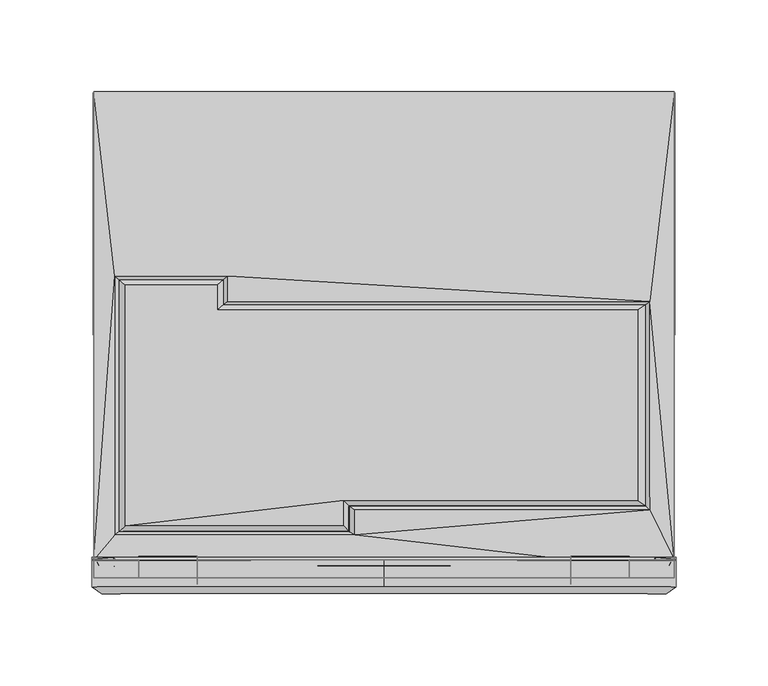
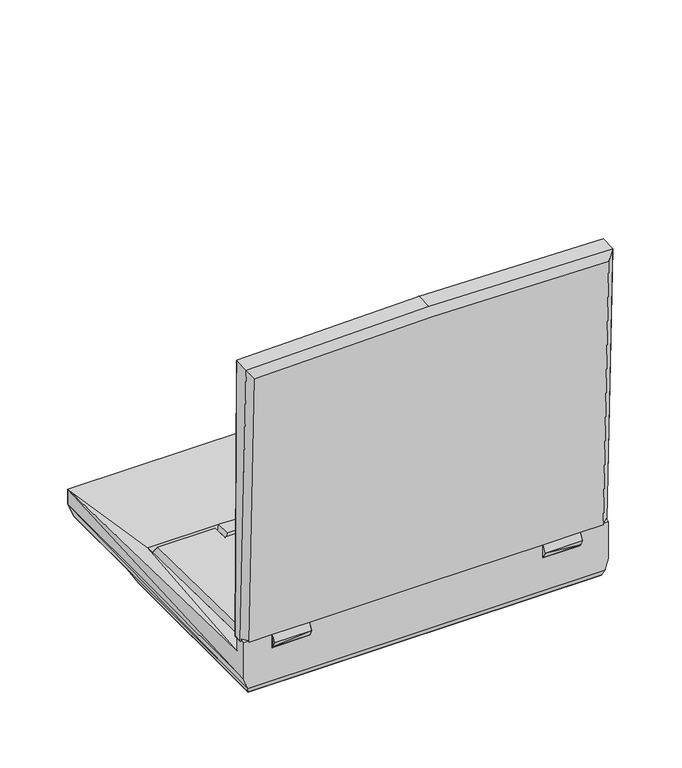
"""IFC4 building model written with IfcOpenShell, lengths in millimetres: proxy geometry, Entourage_RPC_Notebook_Computer : Entourage_RPC_Notebook_Computer."""

import ifcopenshell
import ifcopenshell.guid

model = None  # the IFC model being written
_history = None  # IfcOwnerHistory: only IFC2X3 demands one
_inside = {}  # id of a spatial element -> (the spatial element, [elements in it])
_under = {}  # id of a project, library or spatial element -> (it, [spatial elements below it])
_declared = {}  # id of a project -> (the project, [libraries it declares])
_typed = {}  # id of a type object -> (the type object, [elements of that type])
_made_of = {}  # id of a material, layer set ... -> (it, [elements and type objects made of it])


def new_model(schema):
    """Start an empty IFC model of exactly this schema.

    Asked for "IFC4X3", IfcOpenShell would pick the latest addendum, in which some entities
    have other attributes; the version numbers below select the first issue.
    IFC2X3 requires an IfcOwnerHistory on every rooted entity: one is made here for all.
    """
    global model, _history
    if schema == "IFC4X3":
        model = ifcopenshell.file(schema_version=(4, 3, 0, 0))
    else:
        model = ifcopenshell.file(schema=schema)
    _inside.clear()
    _under.clear()
    _declared.clear()
    _typed.clear()
    _made_of.clear()
    _history = None
    if model.schema == "IFC2X3":
        org = make("IfcOrganization", Name="unknown")
        user = make(
            "IfcPersonAndOrganization",
            ThePerson=make("IfcPerson", FamilyName="unknown"),
            TheOrganization=org,
        )
        app = make(
            "IfcApplication",
            ApplicationDeveloper=org,
            Version="unknown",
            ApplicationFullName="unknown",
            ApplicationIdentifier="unknown",
        )
        _history = make(
            "IfcOwnerHistory",
            OwningUser=user,
            OwningApplication=app,
            ChangeAction="ADDED",
            CreationDate=0,
        )
    return model


def make(cls, **values):
    """One entity of the class cls with the attributes given. An attribute that is None is left unset."""
    return model.create_entity(
        cls, **{name: value for name, value in values.items() if value is not None}
    )


def rooted(cls, **values):
    """An entity with a GlobalId (a new one), such as an element, a storey or a relation."""
    return make(cls, GlobalId=ifcopenshell.guid.new(), OwnerHistory=_history, **values)


def si_unit(unit_type, name, prefix=None):
    """IfcSIUnit, for example si_unit("LENGTHUNIT", "METRE", prefix="MILLI")."""
    return make("IfcSIUnit", UnitType=unit_type, Prefix=prefix, Name=name)


def assignment(units):
    """IfcUnitAssignment: the units of a project."""
    return None if units is None else make("IfcUnitAssignment", Units=units)


def point(xyz):
    """IfcCartesianPoint."""
    return None if xyz is None else make("IfcCartesianPoint", Coordinates=xyz)


def direction(xyz):
    """IfcDirection."""
    return None if xyz is None else make("IfcDirection", DirectionRatios=xyz)


def frame(location, z_axis=None, x_axis=None):
    """IfcAxis2Placement3D, a coordinate frame: its origin and axes. An axis left out is left unset."""
    return make(
        "IfcAxis2Placement3D",
        Location=point(location),
        Axis=direction(z_axis),
        RefDirection=direction(x_axis),
    )


def origin():
    """The frame at (0, 0, 0) with its axes left unset."""
    return frame((0.0, 0.0, 0.0))


def place(relative_to, where):
    """IfcLocalPlacement: puts the frame where relative to a parent placement (None: the world)."""
    return make(
        "IfcLocalPlacement", PlacementRelTo=relative_to, RelativePlacement=where
    )


def context(
    kind, dimensions, precision=None, world=None, true_north=None, identifier=None
):
    """IfcGeometricRepresentationContext, for example the 3D "Model" context."""
    return make(
        "IfcGeometricRepresentationContext",
        ContextIdentifier=identifier,
        ContextType=kind,
        CoordinateSpaceDimension=dimensions,
        Precision=precision,
        WorldCoordinateSystem=world,
        TrueNorth=true_north,
    )


def project(units=None, contexts=None):
    """IfcProject with its units and contexts."""
    return rooted(
        "IfcProject",
        Name="project",
        RepresentationContexts=contexts,
        UnitsInContext=assignment(units),
    )


def spatial(cls, under=None, at=None, **own):
    """A site, building, storey or space (cls), placed at a placement, below another one or the project."""
    s = rooted(cls, ObjectPlacement=at, **own)
    if under is not None:
        _under.setdefault(under.id(), (under, []))[1].append(s)
    return s


def point_list(points):
    """IfcCartesianPointList2D or 3D."""
    cls = (
        "IfcCartesianPointList2D" if len(points[0]) == 2 else "IfcCartesianPointList3D"
    )
    return make(cls, CoordList=points)


def triangles(points, corners, closed=None, point_numbers=None):
    """IfcTriangulatedFaceSet: each triangle names its three corners, points numbered from 1."""
    return make(
        "IfcTriangulatedFaceSet",
        Coordinates=point_list(points),
        Closed=closed,
        CoordIndex=corners,
        PnIndex=point_numbers,
    )


def shape(context_of_items, identifier, shape_type, items):
    """IfcShapeRepresentation: the items that make up one representation, for example the "Body"."""
    return make(
        "IfcShapeRepresentation",
        ContextOfItems=context_of_items,
        RepresentationIdentifier=identifier,
        RepresentationType=shape_type,
        Items=items,
    )


def source(mapping_origin, context_of_items, identifier, shape_type, items):
    """IfcRepresentationMap: a shape defined once, which mapped items show again and again."""
    return make(
        "IfcRepresentationMap",
        MappingOrigin=mapping_origin,
        MappedRepresentation=shape(context_of_items, identifier, shape_type, items),
    )


def transform(
    local_origin,
    x_axis=None,
    y_axis=None,
    z_axis=None,
    scale=None,
    scale2=None,
    scale3=None,
    uniform=True,
):
    """IfcCartesianTransformationOperator3D, or its non-uniform kind. x_axis, y_axis, z_axis: its Axis1, 2, 3."""
    if uniform:
        return make(
            "IfcCartesianTransformationOperator3D",
            Axis1=direction(x_axis),
            Axis2=direction(y_axis),
            LocalOrigin=point(local_origin),
            Scale=scale,
            Axis3=direction(z_axis),
        )
    return make(
        "IfcCartesianTransformationOperator3DnonUniform",
        Axis1=direction(x_axis),
        Axis2=direction(y_axis),
        LocalOrigin=point(local_origin),
        Scale=scale,
        Axis3=direction(z_axis),
        Scale2=scale2,
        Scale3=scale3,
    )


def mapped(mapping_source, mapping_target):
    """IfcMappedItem: shows the shape of a source again, moved by a transform."""
    return make(
        "IfcMappedItem", MappingSource=mapping_source, MappingTarget=mapping_target
    )


def made_of(thing, what):
    """Note that an element or type object is made of a material, layer set ...; save() writes the relation."""
    if what is not None:
        _made_of.setdefault(what.id(), (what, []))[1].append(thing)
    return thing


def element(
    cls,
    number,
    at=None,
    inside=None,
    cuts=None,
    type_object=None,
    material=None,
    context=None,
    identifier="Body",
    shape_type=None,
    held_by="IfcProductDefinitionShape",
    body=None,
    shapes=None,
    **own,
):
    """One element of the class cls, such as IfcWall. Its Tag is "e" and its number.

    at: its placement. inside: the storey or other place that contains it. cuts: it is an
    opening in that element (IfcRelVoidsElement). A single representation is given by context,
    identifier, shape_type and body (its items); several are given by shapes. held_by: the class
    of the entity that holds the representations. save() writes the other relations.
    """
    e = rooted(cls, Tag="e%d" % number, ObjectPlacement=at, **own)
    if body is not None:
        shapes = [shape(context, identifier, shape_type, body)]
    if shapes is not None:
        e.Representation = make(held_by, Representations=shapes)
    if inside is not None:
        _inside.setdefault(inside.id(), (inside, []))[1].append(e)
    if cuts is not None:
        rooted(
            "IfcRelVoidsElement", RelatingBuildingElement=cuts, RelatedOpeningElement=e
        )
    if type_object is not None:
        _typed.setdefault(type_object.id(), (type_object, []))[1].append(e)
    return made_of(e, material)


def aggregate(whole, parts):
    """IfcRelAggregates: a whole, such as a stair, and the parts it consists of."""
    return rooted("IfcRelAggregates", RelatingObject=whole, RelatedObjects=parts)


def save(model, path):
    """Write the relations noted so far, then the file.

    IfcRelAggregates (storeys below a building ...), IfcRelContainedInSpatialStructure (elements
    in a storey), IfcRelDefinesByType, IfcRelAssociatesMaterial and IfcRelDeclares: one each for
    every whole, place, type object, material and project.
    """
    for whole, parts in _under.values():
        aggregate(whole, parts)
    for where, things in _inside.values():
        rooted(
            "IfcRelContainedInSpatialStructure",
            RelatedElements=things,
            RelatingStructure=where,
        )
    for kind, things in _typed.values():
        rooted("IfcRelDefinesByType", RelatedObjects=things, RelatingType=kind)
    for what, things in _made_of.values():
        rooted("IfcRelAssociatesMaterial", RelatedObjects=things, RelatingMaterial=what)
    for by, libraries in _declared.values():
        rooted("IfcRelDeclares", RelatingContext=by, RelatedDefinitions=libraries)
    model.write(path)


def entourage_8896f287(model_context):
    return source(origin(), model_context, "Body", "Tessellation", [
        triangles([(158.4296647, 167.5812681, 28.2218875), (101.7496669, -97.7313983, 35.1332139), (101.7496669, -97.7313983, 48.4910491), (101.7496669, -92.7961799, 50.2665039), (101.7496669, -87.9168539, 48.1837095), (101.7496669, -87.9168539, 35.1332139), (158.4296647, -87.9168539, 35.1332139), (133.8221823, -97.7288549, 35.1332139), (133.8221823, -97.7313983, 48.4910491), (133.8221823, -92.7961799, 50.2665039), (133.8221823, -87.9168539, 48.1837095), (133.8221823, -87.9168539, 35.1332139), (-158.4322081, 167.5812681, 28.2218875), (-101.7496669, -97.7313983, 35.1332139), (-101.7496669, -97.7313983, 48.4910491), (-101.7496669, -92.7961799, 50.2665039), (-101.7496669, -87.9168539, 48.1837095), (-101.7496669, -87.9168539, 35.1332139), (-85.2320795, 66.8399745, 31.8083601), (144.8813274, 53.1646373, 31.9658404), (-85.2320795, 53.1646373, 31.9658404), (144.8813274, -60.6703247, 34.190875), (-146.9209376, -74.3380406, 34.2924744), (-146.9209376, 66.8399745, 31.8083601), (-158.4322081, -87.9168539, 35.1332139), (-133.8247257, -97.7313983, 35.1332139), (-133.8247257, -97.7313983, 48.4910491), (-133.8247257, -92.7961799, 50.2665039), (-133.8247257, -87.9168539, 48.1837095), (-133.8247257, -87.9168539, 35.1332139), (142.7070869, -58.4935499, 29.3902845), (-15.8851303, -74.3380406, 34.2924744), (-19.0347234, -72.5752803, 29.491884), (-15.8851303, -60.6703247, 34.190875), (-19.0347234, -58.4935499, 29.3902845), (155.2851437, 164.0506697, 4.7853507), (155.2851437, 83.3296248, 4.869171), (153.4715916, 69.0040502, 0.0), (153.4715916, -95.8771965, 0.0), (-155.2876871, 164.0506697, 4.7853507), (-155.2851437, 83.3296248, 4.869171), (-153.4715916, 69.0040502, 0.0), (-153.4715916, -95.8771965, 0.0), (155.2851437, -97.7313983, 4.869171), (158.4296647, -97.7313983, 14.9046918), (158.4296647, -97.7313983, 48.4910491), (-155.2851437, -97.7313983, 4.869171), (-158.4322081, -97.7313983, 14.9046918), (-158.4322081, -97.7313983, 48.4910491), (158.4296647, -92.7961799, 50.2665039), (158.4296647, -87.9168539, 48.1837095), (-158.4322081, -92.7961799, 50.2665039), (-158.4322081, -87.9168539, 48.1837095), (158.6201509, 166.809095, 14.9046918), (-158.6201509, 166.809095, 14.9046918), (-87.4063109, 64.9654568, 27.0992089), (142.7070869, 51.2901242, 27.2541481), (-87.4063109, 51.2901242, 27.2541481), (-144.7467062, -72.5752803, 29.491884), (-144.7467062, 64.9654568, 27.0992089), (-141.2262725, 62.1181243, 32.971677), (-90.9267446, 62.1181243, 32.971677), (138.3738576, 48.4427871, 33.1266163), (-90.9267446, 48.4427871, 33.1266163), (138.3738576, -55.455713, 35.1128935), (-141.2262725, -69.5374479, 35.2170342), (-21.8820582, -55.455713, 35.1128935), (-21.8820582, -69.5374479, 35.2170342), (0.0, -90.1722394, 56.3506665), (0.0, -94.0301344, 283.6618462), (145.6915886, -90.167307, 56.3494402), (145.6915886, -94.0301344, 283.6618462), (-145.109929, -90.167307, 56.3494402), (-145.109929, -94.0301344, 283.6618462), (0.0, -86.6469732, 54.9193722), (0.0, -90.9261269, 284.9821508), (147.9064607, -86.6414321, 54.9206076), (147.9064607, -90.9261269, 284.9821508), (-147.3248011, -86.6414321, 54.9206076), (-147.3248011, -90.9261269, 284.9821508), (0.0, -88.1607071, 305.3969839), (0.0, -102.413053, 304.8563192), (159.4431202, -88.386847, 302.5685955), (159.4431202, -102.6416636, 302.0285485), (-159.4431202, -88.386847, 302.5685955), (-159.4431202, -102.6416636, 302.0285485), (0.0, -106.3485413, 297.4293198), (0.0, -98.2380444, 47.5817886), (101.7496669, -99.2864996, 36.8041307), (154.0176883, -106.5746903, 294.6009314), (101.7496669, -98.2380444, 47.5817886), (133.8221823, -99.2729467, 36.8059883), (133.7332887, -98.2380444, 47.5817886), (154.0176883, -98.2380444, 47.5817886), (133.8221823, -101.2159331, 41.6751679), (101.7496669, -101.2159331, 41.6751679), (159.4431202, -94.0607739, 47.7261203), (-101.7496669, -99.2864996, 36.8041307), (-154.0176883, -106.5746903, 294.6009314), (-101.7496669, -98.2380444, 47.5817886), (-133.8221823, -99.2729467, 36.8059883), (-133.7332887, -98.2380444, 47.5817886), (-154.0176883, -98.2380444, 47.5817886), (-133.8221823, -101.2159331, 41.6751679), (-101.7496669, -101.2159331, 41.6751679), (-159.4431202, -94.0607739, 47.7261203), (0.0, -86.4984357, 47.9871781), (101.7496669, -85.924897, 37.2684533), (101.7496669, -86.5033682, 47.9884044), (133.8221823, -85.924897, 37.2684533), (-101.7496669, -85.924897, 37.2684533), (-101.7496669, -86.5033682, 47.9884044), (-133.8221823, -85.924897, 37.2684533), (133.7332887, -86.5033682, 47.9884044), (159.4431202, -86.4953563, 47.9890267), (-133.7332887, -86.5033682, 47.9884044), (-159.4431202, -86.4953563, 47.9890267), (0.0, -88.1641952, 303.1256291), (156.9437634, -88.3928059, 300.2978765), (159.4431202, -87.6648889, 205.2385081), (0.0, -91.14827, 301.1419566), (155.5010462, -91.376263, 298.3166385), (-156.9437634, -88.3928059, 300.2978765), (-159.4431202, -87.6648889, 205.2385081), (-155.5010462, -91.376263, 298.3166385)], [[19, 1, 13], [2, 6, 3], [3, 6, 4], [4, 6, 5], [12, 6, 8], [8, 6, 2], [11, 12, 10], [10, 12, 9], [9, 12, 8], [21, 20, 19], [20, 1, 19], [22, 6, 12], [1, 20, 7], [22, 12, 7], [23, 6, 32], [18, 6, 23], [19, 13, 24], [14, 15, 18], [15, 16, 18], [16, 17, 18], [30, 26, 18], [26, 14, 18], [29, 28, 30], [28, 27, 30], [27, 26, 30], [24, 25, 23], [23, 30, 18], [13, 25, 24], [23, 25, 30], [32, 6, 22], [22, 34, 32], [31, 33, 35], [37, 41, 36], [36, 41, 40], [42, 41, 38], [38, 41, 37], [39, 43, 38], [38, 43, 42], [44, 8, 2], [8, 44, 45], [45, 46, 9], [9, 8, 45], [44, 47, 39], [39, 47, 43], [2, 14, 47], [2, 47, 44], [3, 15, 14], [3, 14, 2], [47, 14, 26], [26, 48, 47], [48, 27, 49], [27, 48, 26], [50, 51, 11], [11, 10, 50], [5, 17, 16], [5, 16, 4], [52, 29, 53], [29, 52, 28], [46, 50, 10], [10, 9, 46], [4, 16, 15], [4, 15, 3], [49, 28, 52], [28, 49, 27], [13, 1, 55], [55, 1, 54], [55, 54, 40], [40, 54, 36], [55, 40, 41], [48, 52, 25], [52, 48, 49], [53, 25, 52], [41, 43, 47], [13, 48, 25], [55, 47, 48], [43, 41, 42], [48, 13, 55], [47, 55, 41], [51, 7, 12], [12, 11, 51], [6, 18, 17], [6, 17, 5], [53, 30, 25], [30, 53, 29], [54, 37, 36], [45, 7, 50], [50, 46, 45], [51, 50, 7], [37, 44, 39], [1, 7, 45], [54, 45, 44], [39, 38, 37], [45, 54, 1], [44, 37, 54], [57, 31, 22], [23, 32, 33], [33, 59, 23], [20, 21, 58], [58, 57, 20], [21, 19, 56], [56, 58, 21], [19, 24, 60], [60, 56, 19], [24, 23, 59], [59, 60, 24], [34, 22, 31], [31, 35, 34], [33, 32, 34], [34, 35, 33], [59, 35, 33], [20, 22, 7], [22, 20, 57], [67, 65, 63], [67, 63, 64], [64, 62, 61], [66, 64, 61], [31, 57, 63], [63, 65, 31], [35, 31, 65], [65, 67, 35], [57, 58, 64], [64, 63, 57], [58, 56, 62], [62, 64, 58], [56, 60, 61], [61, 62, 56], [60, 59, 66], [66, 61, 60], [66, 67, 64], [68, 66, 59], [59, 33, 68], [35, 67, 68], [68, 33, 35], [66, 68, 67], [69, 70, 72], [69, 72, 71], [69, 74, 70], [69, 73, 74], [76, 78, 72], [72, 70, 76], [77, 75, 69], [69, 71, 77], [78, 77, 71], [71, 72, 78], [76, 74, 80], [74, 76, 70], [79, 69, 75], [69, 79, 73], [80, 73, 79], [73, 80, 74], [81, 82, 84], [81, 84, 83], [81, 86, 82], [81, 85, 86], [82, 87, 90], [82, 90, 84], [87, 88, 91], [87, 91, 90], [90, 91, 93], [96, 89, 92], [96, 92, 95], [90, 93, 94], [97, 90, 94], [91, 95, 93], [91, 96, 95], [97, 84, 90], [82, 99, 87], [82, 86, 99], [87, 100, 88], [87, 99, 100], [99, 102, 100], [105, 101, 98], [105, 104, 101], [102, 99, 103], [106, 103, 99], [100, 102, 104], [100, 104, 105], [106, 99, 86], [89, 108, 110], [89, 110, 92], [96, 91, 89], [89, 91, 108], [108, 91, 109], [91, 88, 109], [109, 88, 107], [98, 113, 111], [98, 101, 113], [105, 98, 100], [98, 111, 100], [111, 112, 100], [100, 112, 88], [112, 107, 88], [93, 114, 115], [93, 115, 97], [95, 92, 93], [93, 92, 114], [114, 92, 110], [93, 97, 94], [102, 117, 116], [102, 106, 117], [104, 102, 101], [102, 116, 101], [116, 113, 101], [102, 103, 106], [108, 109, 114], [108, 114, 110], [81, 83, 119], [109, 107, 75], [75, 77, 109], [114, 109, 77], [120, 115, 77], [114, 77, 115], [119, 118, 81], [77, 78, 120], [119, 120, 122], [76, 121, 122], [76, 122, 78], [119, 122, 121], [119, 121, 118], [120, 78, 122], [83, 120, 119], [111, 116, 112], [111, 113, 116], [81, 123, 85], [112, 75, 107], [75, 112, 79], [116, 79, 112], [124, 79, 117], [117, 79, 116], [123, 81, 118], [79, 124, 80], [123, 125, 124], [76, 125, 121], [76, 80, 125], [123, 121, 125], [123, 118, 121], [124, 125, 80], [85, 123, 124], [117, 86, 124], [117, 106, 86], [124, 86, 85], [115, 120, 84], [115, 84, 97], [120, 83, 84]], closed=False),
    ])


if __name__ == "__main__":
    model = new_model("IFC4")
    model_context = context("Model", 3, world=origin())
    ifc_project = project(units=[si_unit("LENGTHUNIT", "METRE", prefix="MILLI")], contexts=[model_context])
    site = spatial("IfcSite", under=ifc_project)
    building = spatial("IfcBuilding", under=site)
    placement = place(None, origin())
    entourage_shape = entourage_8896f287(model_context)
    element("IfcBuildingElementProxy", 1, Name="Entourage_RPC_Notebook_Computer : Entourage_RPC_Notebook_Computer", ObjectType="Entourage_RPC_Notebook_Computer : Entourage_RPC_Notebook_Computer", at=placement, inside=building, context=model_context, shape_type="MappedRepresentation", body=[
        mapped(entourage_shape, transform((0.0, 0.0, 0.0), x_axis=(1.0, 0.0, 0.0), y_axis=(0.0, 1.0, 0.0), z_axis=(0.0, 0.0, 1.0))),
    ])
    save(model, "model.ifc")

# Revit data of these elements
# Type "Entourage_RPC_Notebook_Computer : Entourage_RPC_Notebook_Computer"
#   built-in parameter 1005198 = "{2, 15},{39, RPC-16-N04H-AQSP-D1N4-43SU-6GKQ-C3KU-1C},{1, 0},{1, 0},{2, 33},{1, 8},{5, Color},{1, 0},{1, 0},{3, 0.8},{3, 0.8},{3, 0.8},{1, 8},{7, BBoxMin},{1, 0},{1, 0},{1, 0},{1, 0},{1, 0},{1, 8},{7, BBoxMax},{1, 0},{1, 0},{1, 0},{1, 0},{1, 0},{2, 11},{9, RPCTypeId},{1, 0},{1, 0},{39, RPC-16-N04H-AQSP-D1N4-43SU-6GKQ-C3KU-1C},{1, 6},{14, RPCPlantHeight},{1, 0},{1, 0},{7, 2.28517},{2, 11},{20, AdvancedUIDefinition},{1, 0},{1, 0},{0, },{2, 11},{10, AssetLibID},{1, 0},{1, 0},{36, 4D3F6E72-3F99-4203-98E9-AF80B3C7A7A4},{2, 11},{10, BaseSchema},{1, 0},{1, 0},{9, RPCSchema},{1, 2},{6, Hidden},{1, 0},{1, 0},{1, 0},{2, 11},{12, LocalizedUID},{1, 0},{1, 0},{0, },{1, 4},{11, RPCCategory},{1, 0},{1, 0},{1, 0},{2, 11},{8, RPCImage},{1, 0},{1, 0},{0, },{1, 4},{13, SchemaVersion},{1, 0},{1, 0},{1, 3},{2, 11},{12, UIDefinition},{1, 0},{1, 0},{0, },{2, 11},{6, UIName},{1, 0},{1, 0},{39, RPC-16-N04H-AQSP-D1N4-43SU-6GKQ-C3KU-1C},{2, 11},{11, VersionGUID},{1, 0},{1, 0},{9, RPCSchema},{2, 11},{9, assettype},{1, 0},{1, 0},{11, RPCGeometry},{2, 11},{11, description},{1, 0},{1, 0},{0, },{2, 11},{9, localname},{1, 0},{1, 0},{3, RPC},{2, 11},{9, localtype},{1, 0},{1, 0},{3, RPC},{1, 4},{8, revision},{1, 0},{1, 0},{1, 1},{2, 11},{9, thumbnail},{1, 0},{1, 0},{0, },{1, 4},{7, version},{1, 0},{1, 0},{1, 1},{2, 14},{6, Height},{1, 0},{1, 0},{7, 2.28517},{1, 2},{20, RPC_Cast Reflections},{1, 0},{1, 0},{1, 0},{1, 4},{8, RPC_Open},{1, 0},{1, 0},{3, -14},{1, 2},{9, RPC_Power},{1, 0},{1, 0},{1, 1},{2, 11},{18, RPC_Screen Preview},{1, 0},{1, 0},{70, __RPC:/object data/textures/object/Top/TopScreen/textures/on/rgb/0/0/0},{2, 11},{20, RPC_i_Screen Preview},{1, 0},{1, 0},{0, },{1, 2},{17, RPC_Custom Screen},{1, 0},{1, 0},{1, 1},{2, 11},{20, RPC_Screen File Name},{1, 0},{1, 0},{56, C:\\Users\\Mary\\Desktop\\Photos\\Brian Aug 2013\\Castle 1.jpg},{2, 11},{7, keyword},{1, 0},{1, 0},{31, :Geometry:RPC:Notebook Computer},{2, 11},{8, category},{1, 0},{1, 0},{15, :Office Clutter},{21, assetlibrary_base.fbx},{1, 5},"
#   built-in parameter 1005195 = "RPC-16-N04H-AQSP-D1N4-43SU-6GKQ-C3KU-1C"
#   Height = 0
